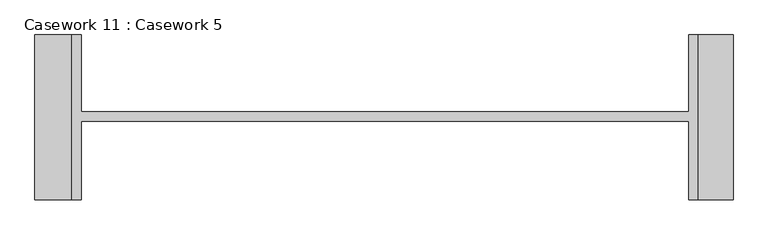
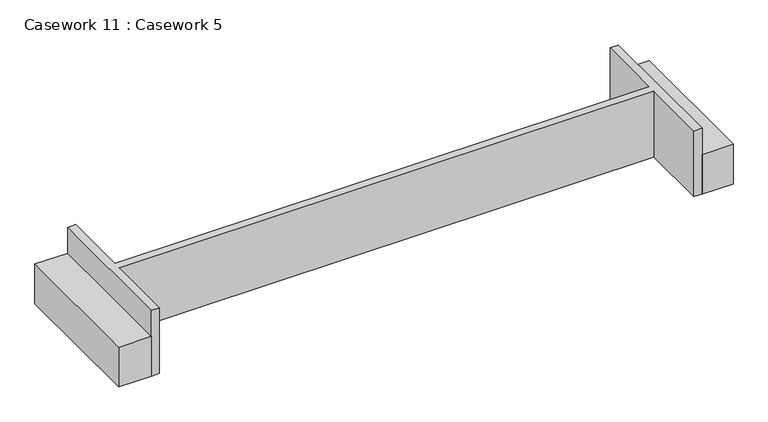
"""IFC4 building model written with IfcOpenShell, lengths in millimetres: furniture geometry, Casework 11 : Casework 5."""

from ifc_helpers import new_model, si_unit, origin, origin_with_axes, place, context, project, spatial, polyline, outline, extrude, source, transform, mapped, element, save


def casework_11_casework_5_901fcd52(model_context):
    return source(origin(), model_context, "Body", "SweptSolid", [
        extrude(outline(polyline([(-45222.23615, 268708.5951951), (-45222.23615, 266167.5438856), (-45765.6431786, 266167.5438856), (-45765.6431786, 268708.5951951), (-45222.23615, 268708.5951951)])), origin_with_axes(), (0.0, 0.0, 1.0), 736.6),
        extrude(outline(polyline([(-55407.3218514, 268708.5951951), (-55407.3218514, 266167.5438856), (-55978.0010565, 266167.5438856), (-55978.0010565, 268708.5951951), (-55407.3218514, 268708.5951951)])), origin_with_axes(), (0.0, 0.0, 1.0), 736.6),
        extrude(outline(polyline([(-55264.4443999, 268708.5951951), (-55264.4443999, 267521.3866807), (-45907.3606126, 267521.3866807), (-45907.3606126, 268708.5951951), (-45765.6431786, 268708.5951951), (-45765.6431786, 266167.5438856), (-45907.3606126, 266167.5438856), (-45907.3606126, 267379.5233622), (-55264.4443999, 267379.5233622), (-55264.4443999, 266167.5438856), (-55407.3218514, 266167.5438856), (-55407.3218514, 268708.5951951), (-55264.4443999, 268708.5951951)])), origin_with_axes(), (0.0, 0.0, 1.0), 1219.2),
    ])


if __name__ == "__main__":
    model = new_model("IFC4")
    model_context = context("Model", 3, world=origin())
    ifc_project = project(units=[si_unit("LENGTHUNIT", "METRE", prefix="MILLI")], contexts=[model_context])
    site = spatial("IfcSite", under=ifc_project)
    building = spatial("IfcBuilding", under=site)
    placement = place(None, origin())
    casework_11_casework_5_shape = casework_11_casework_5_901fcd52(model_context)
    element("IfcFurniture", 1, ObjectType="Casework 11 : Casework 5", at=placement, inside=building, context=model_context, shape_type="MappedRepresentation", body=[
        mapped(casework_11_casework_5_shape, transform((0.0, 0.0, 0.0), x_axis=(1.0, 0.0, 0.0), y_axis=(0.0, 1.0, 0.0), z_axis=(0.0, 0.0, 1.0))),
    ])
    save(model, "model.ifc")

# Revit data of these elements
# Element 1 (IfcFurniture, "Casework 11 : Casework 5")
#   Materials on its faces: "WOOD VENEER"
# Materials
#   "WOOD VENEER": class "Miscellaneous", colour RGB 164 164 164, transparency 0, Cost = 0
